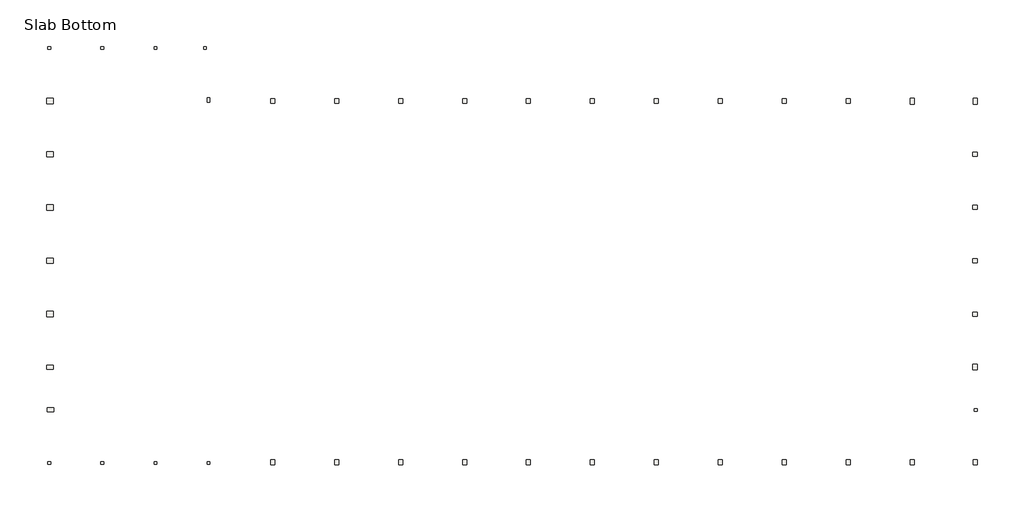
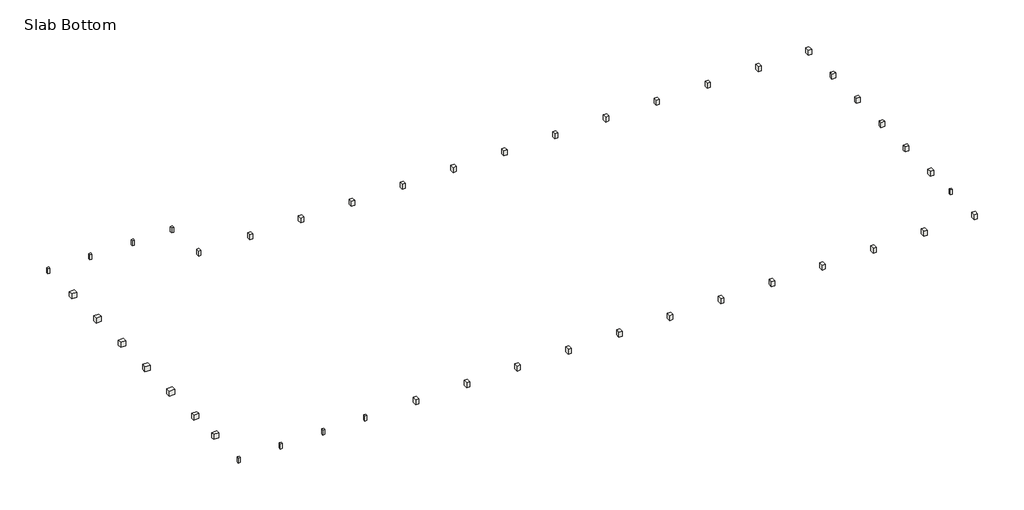
# One storey: 46 slabs.
"""IFC4 building model written with IfcOpenShell, lengths in millimetres."""

from ifc_helpers import new_model, si_unit, frame, origin, place, context, project, spatial, polyline, outline, extrude, element, save

model = new_model("IFC4")

# Units and contexts
model_context = context("Model", 3, world=origin())
ifc_project = project(units=[si_unit("LENGTHUNIT", "METRE", prefix="MILLI")], contexts=[model_context])

# Site, building, storey
site = spatial("IfcSite", under=ifc_project)
building = spatial("IfcBuilding", under=site)
storey = spatial("IfcBuildingStorey", under=building, Name="Slab Bottom", Elevation=-152.4)

# Slabs
placement = place(None, origin())
element("IfcSlab", 1, ObjectType="Footing-Rectangular : P1", at=placement, inside=storey, context=model_context, shape_type="SweptSolid", body=[
    extrude(outline(polyline([(304747.7148264, -530797.8413841), (305052.5148264, -530797.8413841), (305052.5148264, -531102.6413841), (304747.7148264, -531102.6413841), (304747.7148264, -530797.8413841)])), frame((0.0, 0.0, -1066.8), z_axis=(0.0, 0.0, 1.0), x_axis=(1.0, 0.0, 0.0)), (0.0, 0.0, 1.0), 762.0),
])
element("IfcSlab", 2, ObjectType="Footing-Rectangular : P1", at=placement, inside=storey, context=model_context, shape_type="SweptSolid", body=[
    extrude(outline(polyline([(310840.5398264, -530801.0163841), (311145.3398264, -530801.0163841), (311145.3398264, -531105.8163841), (310840.5398264, -531105.8163841), (310840.5398264, -530801.0163841)])), frame((0.0, 0.0, -1066.8), z_axis=(0.0, 0.0, 1.0), x_axis=(1.0, 0.0, 0.0)), (0.0, 0.0, 1.0), 762.0),
])
element("IfcSlab", 3, ObjectType="Footing-Rectangular : P1", at=placement, inside=storey, context=model_context, shape_type="SweptSolid", body=[
    extrude(outline(polyline([(316968.2898264, -530801.0163841), (317273.0898264, -530801.0163841), (317273.0898264, -531105.8163841), (316968.2898264, -531105.8163841), (316968.2898264, -530801.0163841)])), frame((0.0, 0.0, -1066.8), z_axis=(0.0, 0.0, 1.0), x_axis=(1.0, 0.0, 0.0)), (0.0, 0.0, 1.0), 762.0),
])
element("IfcSlab", 4, ObjectType="Footing-Rectangular : P1", at=placement, inside=storey, context=model_context, shape_type="SweptSolid", body=[
    extrude(outline(polyline([(322661.0648264, -531102.6413841), (322661.0648264, -530797.8413841), (322965.8648264, -530797.8413841), (322965.8648264, -531102.6413841), (322661.0648264, -531102.6413841)])), frame((0.0, 0.0, -1066.8), z_axis=(0.0, 0.0, 1.0), x_axis=(1.0, 0.0, 0.0)), (0.0, 0.0, 1.0), 762.0),
])
element("IfcSlab", 5, ObjectType="Footing-Rectangular : P1", at=placement, inside=storey, context=model_context, shape_type="SweptSolid", body=[
    extrude(outline(polyline([(304741.3648264, -578543.4913841), (305046.1648264, -578543.4913841), (305046.1648264, -578848.2913841), (304741.3648264, -578848.2913841), (304741.3648264, -578543.4913841)])), frame((0.0, 0.0, -1066.8), z_axis=(0.0, 0.0, 1.0), x_axis=(1.0, 0.0, 0.0)), (0.0, 0.0, 1.0), 762.0),
])
element("IfcSlab", 6, ObjectType="Footing-Rectangular : P1", at=placement, inside=storey, context=model_context, shape_type="SweptSolid", body=[
    extrude(outline(polyline([(310840.5398264, -578845.1163841), (310840.5398264, -578540.3163841), (311145.3398264, -578540.3163841), (311145.3398264, -578845.1163841), (310840.5398264, -578845.1163841)])), frame((0.0, 0.0, -1066.8), z_axis=(0.0, 0.0, 1.0), x_axis=(1.0, 0.0, 0.0)), (0.0, 0.0, 1.0), 762.0),
])
element("IfcSlab", 7, ObjectType="Footing-Rectangular : P1", at=placement, inside=storey, context=model_context, shape_type="SweptSolid", body=[
    extrude(outline(polyline([(316971.4648264, -578845.1163841), (316971.4648264, -578540.3163841), (317276.2648264, -578540.3163841), (317276.2648264, -578845.1163841), (316971.4648264, -578845.1163841)])), frame((0.0, 0.0, -1066.8), z_axis=(0.0, 0.0, 1.0), x_axis=(1.0, 0.0, 0.0)), (0.0, 0.0, 1.0), 762.0),
])
element("IfcSlab", 8, ObjectType="Footing-Rectangular : P1", at=placement, inside=storey, context=model_context, shape_type="SweptSolid", body=[
    extrude(outline(polyline([(323067.4648264, -578543.4913841), (323372.2648264, -578543.4913841), (323372.2648264, -578848.2913841), (323067.4648264, -578848.2913841), (323067.4648264, -578543.4913841)])), frame((0.0, 0.0, -1066.8), z_axis=(0.0, 0.0, 1.0), x_axis=(1.0, 0.0, 0.0)), (0.0, 0.0, 1.0), 762.0),
])
element("IfcSlab", 9, ObjectType="Footing-Rectangular : P1", at=placement, inside=storey, context=model_context, shape_type="SweptSolid", body=[
    extrude(outline(polyline([(411307.0648264, -572441.1413841), (411611.8648264, -572441.1413841), (411611.8648264, -572745.9413841), (411307.0648264, -572745.9413841), (411307.0648264, -572441.1413841)])), frame((0.0, 0.0, -1066.8), z_axis=(0.0, 0.0, 1.0), x_axis=(1.0, 0.0, 0.0)), (0.0, 0.0, 1.0), 762.0),
])
element("IfcSlab", 10, ObjectType="Footing-Rectangular : P2", at=placement, inside=storey, context=model_context, shape_type="SweptSolid", body=[
    extrude(outline(polyline([(323375.4398264, -536716.0413841), (323375.4398264, -537224.0413841), (323070.6398264, -537224.0413841), (323070.6398264, -536716.0413841), (323375.4398264, -536716.0413841)])), frame((0.0, 0.0, -1066.8), z_axis=(0.0, 0.0, 1.0), x_axis=(1.0, 0.0, 0.0)), (0.0, 0.0, 1.0), 762.0),
])
element("IfcSlab", 11, ObjectType="Footing-Rectangular : P3", at=placement, inside=storey, context=model_context, shape_type="SweptSolid", body=[
    extrude(outline(polyline([(411110.2148264, -561334.9913841), (411643.6148264, -561334.9913841), (411643.6148264, -561792.1913841), (411110.2148264, -561792.1913841), (411110.2148264, -561334.9913841)])), frame((0.0, 0.0, -1066.8), z_axis=(0.0, 0.0, 1.0), x_axis=(1.0, 0.0, 0.0)), (0.0, 0.0, 1.0), 762.0),
])
element("IfcSlab", 12, ObjectType="Footing-Rectangular : P3", at=placement, inside=storey, context=model_context, shape_type="SweptSolid", body=[
    extrude(outline(polyline([(411110.2148264, -555207.2413841), (411643.6148264, -555207.2413841), (411643.6148264, -555664.4413841), (411110.2148264, -555664.4413841), (411110.2148264, -555207.2413841)])), frame((0.0, 0.0, -1066.8), z_axis=(0.0, 0.0, 1.0), x_axis=(1.0, 0.0, 0.0)), (0.0, 0.0, 1.0), 762.0),
])
element("IfcSlab", 13, ObjectType="Footing-Rectangular : P3", at=placement, inside=storey, context=model_context, shape_type="SweptSolid", body=[
    extrude(outline(polyline([(411110.2148264, -549079.4913841), (411643.6148264, -549079.4913841), (411643.6148264, -549536.6913841), (411110.2148264, -549536.6913841), (411110.2148264, -549079.4913841)])), frame((0.0, 0.0, -1066.8), z_axis=(0.0, 0.0, 1.0), x_axis=(1.0, 0.0, 0.0)), (0.0, 0.0, 1.0), 762.0),
])
element("IfcSlab", 14, ObjectType="Footing-Rectangular : P3", at=placement, inside=storey, context=model_context, shape_type="SweptSolid", body=[
    extrude(outline(polyline([(411110.2148264, -542951.7413841), (411643.6148264, -542951.7413841), (411643.6148264, -543408.9413841), (411110.2148264, -543408.9413841), (411110.2148264, -542951.7413841)])), frame((0.0, 0.0, -1066.8), z_axis=(0.0, 0.0, 1.0), x_axis=(1.0, 0.0, 0.0)), (0.0, 0.0, 1.0), 762.0),
])
element("IfcSlab", 15, ObjectType="Footing-Rectangular : P3A", at=placement, inside=storey, context=model_context, shape_type="SweptSolid", body=[
    extrude(outline(polyline([(397010.0398264, -536811.2913841), (397010.0398264, -537344.6913841), (396552.8398264, -537344.6913841), (396552.8398264, -536811.2913841), (397010.0398264, -536811.2913841)])), frame((0.0, 0.0, -1066.8), z_axis=(0.0, 0.0, 1.0), x_axis=(1.0, 0.0, 0.0)), (0.0, 0.0, 1.0), 762.0),
])
element("IfcSlab", 16, ObjectType="Footing-Rectangular : P3A", at=placement, inside=storey, context=model_context, shape_type="SweptSolid", body=[
    extrude(outline(polyline([(389656.7398264, -536811.2913841), (389656.7398264, -537344.6913841), (389199.5398264, -537344.6913841), (389199.5398264, -536811.2913841), (389656.7398264, -536811.2913841)])), frame((0.0, 0.0, -1066.8), z_axis=(0.0, 0.0, 1.0), x_axis=(1.0, 0.0, 0.0)), (0.0, 0.0, 1.0), 762.0),
])
element("IfcSlab", 17, ObjectType="Footing-Rectangular : P3A", at=placement, inside=storey, context=model_context, shape_type="SweptSolid", body=[
    extrude(outline(polyline([(382303.4398264, -536811.2913841), (382303.4398264, -537344.6913841), (381846.2398264, -537344.6913841), (381846.2398264, -536811.2913841), (382303.4398264, -536811.2913841)])), frame((0.0, 0.0, -1066.8), z_axis=(0.0, 0.0, 1.0), x_axis=(1.0, 0.0, 0.0)), (0.0, 0.0, 1.0), 762.0),
])
element("IfcSlab", 18, ObjectType="Footing-Rectangular : P3A", at=placement, inside=storey, context=model_context, shape_type="SweptSolid", body=[
    extrude(outline(polyline([(374950.1398264, -536811.2913841), (374950.1398264, -537344.6913841), (374492.9398264, -537344.6913841), (374492.9398264, -536811.2913841), (374950.1398264, -536811.2913841)])), frame((0.0, 0.0, -1066.8), z_axis=(0.0, 0.0, 1.0), x_axis=(1.0, 0.0, 0.0)), (0.0, 0.0, 1.0), 762.0),
])
element("IfcSlab", 19, ObjectType="Footing-Rectangular : P3A", at=placement, inside=storey, context=model_context, shape_type="SweptSolid", body=[
    extrude(outline(polyline([(367596.8398264, -536811.2913841), (367596.8398264, -537344.6913841), (367139.6398264, -537344.6913841), (367139.6398264, -536811.2913841), (367596.8398264, -536811.2913841)])), frame((0.0, 0.0, -1066.8), z_axis=(0.0, 0.0, 1.0), x_axis=(1.0, 0.0, 0.0)), (0.0, 0.0, 1.0), 762.0),
])
element("IfcSlab", 20, ObjectType="Footing-Rectangular : P3A", at=placement, inside=storey, context=model_context, shape_type="SweptSolid", body=[
    extrude(outline(polyline([(360243.5398264, -536811.2913841), (360243.5398264, -537344.6913841), (359786.3398264, -537344.6913841), (359786.3398264, -536811.2913841), (360243.5398264, -536811.2913841)])), frame((0.0, 0.0, -1066.8), z_axis=(0.0, 0.0, 1.0), x_axis=(1.0, 0.0, 0.0)), (0.0, 0.0, 1.0), 762.0),
])
element("IfcSlab", 21, ObjectType="Footing-Rectangular : P3A", at=placement, inside=storey, context=model_context, shape_type="SweptSolid", body=[
    extrude(outline(polyline([(352890.2398264, -536811.2913841), (352890.2398264, -537344.6913841), (352433.0398264, -537344.6913841), (352433.0398264, -536811.2913841), (352890.2398264, -536811.2913841)])), frame((0.0, 0.0, -1066.8), z_axis=(0.0, 0.0, 1.0), x_axis=(1.0, 0.0, 0.0)), (0.0, 0.0, 1.0), 762.0),
])
element("IfcSlab", 22, ObjectType="Footing-Rectangular : P3A", at=placement, inside=storey, context=model_context, shape_type="SweptSolid", body=[
    extrude(outline(polyline([(345536.9398264, -536811.2913841), (345536.9398264, -537344.6913841), (345079.7398264, -537344.6913841), (345079.7398264, -536811.2913841), (345536.9398264, -536811.2913841)])), frame((0.0, 0.0, -1066.8), z_axis=(0.0, 0.0, 1.0), x_axis=(1.0, 0.0, 0.0)), (0.0, 0.0, 1.0), 762.0),
])
element("IfcSlab", 23, ObjectType="Footing-Rectangular : P3A", at=placement, inside=storey, context=model_context, shape_type="SweptSolid", body=[
    extrude(outline(polyline([(338183.6398264, -536811.2913841), (338183.6398264, -537344.6913841), (337726.4398264, -537344.6913841), (337726.4398264, -536811.2913841), (338183.6398264, -536811.2913841)])), frame((0.0, 0.0, -1066.8), z_axis=(0.0, 0.0, 1.0), x_axis=(1.0, 0.0, 0.0)), (0.0, 0.0, 1.0), 762.0),
])
element("IfcSlab", 24, ObjectType="Footing-Rectangular : P3A", at=placement, inside=storey, context=model_context, shape_type="SweptSolid", body=[
    extrude(outline(polyline([(330830.3398264, -536811.2913841), (330830.3398264, -537344.6913841), (330373.1398264, -537344.6913841), (330373.1398264, -536811.2913841), (330830.3398264, -536811.2913841)])), frame((0.0, 0.0, -1066.8), z_axis=(0.0, 0.0, 1.0), x_axis=(1.0, 0.0, 0.0)), (0.0, 0.0, 1.0), 762.0),
])
element("IfcSlab", 25, ObjectType="Footing-Rectangular : P4", at=placement, inside=storey, context=model_context, shape_type="SweptSolid", body=[
    extrude(outline(polyline([(330830.3398264, -578318.0663841), (330830.3398264, -578927.6663841), (330373.1398264, -578927.6663841), (330373.1398264, -578318.0663841), (330830.3398264, -578318.0663841)])), frame((0.0, 0.0, -1066.8), z_axis=(0.0, 0.0, 1.0), x_axis=(1.0, 0.0, 0.0)), (0.0, 0.0, 1.0), 762.0),
])
element("IfcSlab", 26, ObjectType="Footing-Rectangular : P4", at=placement, inside=storey, context=model_context, shape_type="SweptSolid", body=[
    extrude(outline(polyline([(338183.6398264, -578318.0663841), (338183.6398264, -578927.6663841), (337726.4398264, -578927.6663841), (337726.4398264, -578318.0663841), (338183.6398264, -578318.0663841)])), frame((0.0, 0.0, -1066.8), z_axis=(0.0, 0.0, 1.0), x_axis=(1.0, 0.0, 0.0)), (0.0, 0.0, 1.0), 762.0),
])
element("IfcSlab", 27, ObjectType="Footing-Rectangular : P4", at=placement, inside=storey, context=model_context, shape_type="SweptSolid", body=[
    extrude(outline(polyline([(345536.9398264, -578318.0663841), (345536.9398264, -578927.6663841), (345079.7398264, -578927.6663841), (345079.7398264, -578318.0663841), (345536.9398264, -578318.0663841)])), frame((0.0, 0.0, -1066.8), z_axis=(0.0, 0.0, 1.0), x_axis=(1.0, 0.0, 0.0)), (0.0, 0.0, 1.0), 762.0),
])
element("IfcSlab", 28, ObjectType="Footing-Rectangular : P4", at=placement, inside=storey, context=model_context, shape_type="SweptSolid", body=[
    extrude(outline(polyline([(352890.2398264, -578318.0663841), (352890.2398264, -578927.6663841), (352433.0398264, -578927.6663841), (352433.0398264, -578318.0663841), (352890.2398264, -578318.0663841)])), frame((0.0, 0.0, -1066.8), z_axis=(0.0, 0.0, 1.0), x_axis=(1.0, 0.0, 0.0)), (0.0, 0.0, 1.0), 762.0),
])
element("IfcSlab", 29, ObjectType="Footing-Rectangular : P4", at=placement, inside=storey, context=model_context, shape_type="SweptSolid", body=[
    extrude(outline(polyline([(360243.5398264, -578318.0663841), (360243.5398264, -578927.6663841), (359786.3398264, -578927.6663841), (359786.3398264, -578318.0663841), (360243.5398264, -578318.0663841)])), frame((0.0, 0.0, -1066.8), z_axis=(0.0, 0.0, 1.0), x_axis=(1.0, 0.0, 0.0)), (0.0, 0.0, 1.0), 762.0),
])
element("IfcSlab", 30, ObjectType="Footing-Rectangular : P4", at=placement, inside=storey, context=model_context, shape_type="SweptSolid", body=[
    extrude(outline(polyline([(367596.8398264, -578318.0663841), (367596.8398264, -578927.6663841), (367139.6398264, -578927.6663841), (367139.6398264, -578318.0663841), (367596.8398264, -578318.0663841)])), frame((0.0, 0.0, -1066.8), z_axis=(0.0, 0.0, 1.0), x_axis=(1.0, 0.0, 0.0)), (0.0, 0.0, 1.0), 762.0),
])
element("IfcSlab", 31, ObjectType="Footing-Rectangular : P4", at=placement, inside=storey, context=model_context, shape_type="SweptSolid", body=[
    extrude(outline(polyline([(374950.1398264, -578318.0663841), (374950.1398264, -578927.6663841), (374492.9398264, -578927.6663841), (374492.9398264, -578318.0663841), (374950.1398264, -578318.0663841)])), frame((0.0, 0.0, -1066.8), z_axis=(0.0, 0.0, 1.0), x_axis=(1.0, 0.0, 0.0)), (0.0, 0.0, 1.0), 762.0),
])
element("IfcSlab", 32, ObjectType="Footing-Rectangular : P4", at=placement, inside=storey, context=model_context, shape_type="SweptSolid", body=[
    extrude(outline(polyline([(382303.4398264, -578318.0663841), (382303.4398264, -578927.6663841), (381846.2398264, -578927.6663841), (381846.2398264, -578318.0663841), (382303.4398264, -578318.0663841)])), frame((0.0, 0.0, -1066.8), z_axis=(0.0, 0.0, 1.0), x_axis=(1.0, 0.0, 0.0)), (0.0, 0.0, 1.0), 762.0),
])
element("IfcSlab", 33, ObjectType="Footing-Rectangular : P4", at=placement, inside=storey, context=model_context, shape_type="SweptSolid", body=[
    extrude(outline(polyline([(389656.7398264, -578318.0663841), (389656.7398264, -578927.6663841), (389199.5398264, -578927.6663841), (389199.5398264, -578318.0663841), (389656.7398264, -578318.0663841)])), frame((0.0, 0.0, -1066.8), z_axis=(0.0, 0.0, 1.0), x_axis=(1.0, 0.0, 0.0)), (0.0, 0.0, 1.0), 762.0),
])
element("IfcSlab", 34, ObjectType="Footing-Rectangular : P4", at=placement, inside=storey, context=model_context, shape_type="SweptSolid", body=[
    extrude(outline(polyline([(397010.0398264, -578311.7163841), (397010.0398264, -578921.3163841), (396552.8398264, -578921.3163841), (396552.8398264, -578311.7163841), (397010.0398264, -578311.7163841)])), frame((0.0, 0.0, -1066.8), z_axis=(0.0, 0.0, 1.0), x_axis=(1.0, 0.0, 0.0)), (0.0, 0.0, 1.0), 762.0),
])
element("IfcSlab", 35, ObjectType="Footing-Rectangular : P4A", at=placement, inside=storey, context=model_context, shape_type="SweptSolid", body=[
    extrude(outline(polyline([(404363.3398264, -578311.7163841), (404363.3398264, -578921.3163841), (403906.1398264, -578921.3163841), (403906.1398264, -578311.7163841), (404363.3398264, -578311.7163841)])), frame((0.0, 0.0, -1066.8), z_axis=(0.0, 0.0, 1.0), x_axis=(1.0, 0.0, 0.0)), (0.0, 0.0, 1.0), 762.0),
])
element("IfcSlab", 36, ObjectType="Footing-Rectangular : P4A", at=placement, inside=storey, context=model_context, shape_type="SweptSolid", body=[
    extrude(outline(polyline([(411659.4898264, -578311.7163841), (411659.4898264, -578921.3163841), (411202.2898264, -578921.3163841), (411202.2898264, -578311.7163841), (411659.4898264, -578311.7163841)])), frame((0.0, 0.0, -1066.8), z_axis=(0.0, 0.0, 1.0), x_axis=(1.0, 0.0, 0.0)), (0.0, 0.0, 1.0), 762.0),
])
element("IfcSlab", 37, ObjectType="Footing-Rectangular : P5", at=placement, inside=storey, context=model_context, shape_type="SweptSolid", body=[
    extrude(outline(polyline([(411615.0397781, -536747.7913841), (411615.0397781, -537408.1913841), (411157.8397781, -537408.1913841), (411157.8397781, -536747.7913841), (411615.0397781, -536747.7913841)])), frame((0.0, 0.0, -1066.8), z_axis=(0.0, 0.0, 1.0), x_axis=(1.0, 0.0, 0.0)), (0.0, 0.0, 1.0), 762.0),
])
element("IfcSlab", 38, ObjectType="Footing-Rectangular : P5", at=placement, inside=storey, context=model_context, shape_type="SweptSolid", body=[
    extrude(outline(polyline([(404363.3398264, -536747.7913841), (404363.3398264, -537408.1913841), (403906.1398264, -537408.1913841), (403906.1398264, -536747.7913841), (404363.3398264, -536747.7913841)])), frame((0.0, 0.0, -1066.8), z_axis=(0.0, 0.0, 1.0), x_axis=(1.0, 0.0, 0.0)), (0.0, 0.0, 1.0), 762.0),
])
element("IfcSlab", 39, ObjectType="Footing-Rectangular : P6", at=placement, inside=storey, context=model_context, shape_type="SweptSolid", body=[
    extrude(outline(polyline([(304642.9398264, -572364.9413841), (305404.9398264, -572364.9413841), (305404.9398264, -572822.1413841), (304642.9398264, -572822.1413841), (304642.9398264, -572364.9413841)])), frame((0.0, 0.0, -1066.8), z_axis=(0.0, 0.0, 1.0), x_axis=(1.0, 0.0, 0.0)), (0.0, 0.0, 1.0), 762.0),
])
element("IfcSlab", 40, ObjectType="Footing-Rectangular : P6A", at=placement, inside=storey, context=model_context, shape_type="SweptSolid", body=[
    extrude(outline(polyline([(304585.7898264, -567462.7413841), (305347.7898264, -567462.7413841), (305347.7898264, -567919.9413841), (304585.7898264, -567919.9413841), (304585.7898264, -567462.7413841)])), frame((0.0, 0.0, -1066.8), z_axis=(0.0, 0.0, 1.0), x_axis=(1.0, 0.0, 0.0)), (0.0, 0.0, 1.0), 762.0),
])
element("IfcSlab", 41, ObjectType="Footing-Rectangular : P7", at=placement, inside=storey, context=model_context, shape_type="SweptSolid", body=[
    extrude(outline(polyline([(411640.4398264, -567361.1414082), (411640.4398264, -567970.7414082), (411132.4398264, -567970.7414082), (411132.4398264, -567361.1414082), (411640.4398264, -567361.1414082)])), frame((0.0, 0.0, -1066.8), z_axis=(0.0, 0.0, 1.0), x_axis=(1.0, 0.0, 0.0)), (0.0, 0.0, 1.0), 762.0),
])
element("IfcSlab", 42, ObjectType="Footing-Rectangular : P8", at=placement, inside=storey, context=model_context, shape_type="SweptSolid", body=[
    extrude(outline(polyline([(304585.7898264, -536747.7913841), (305347.7898264, -536747.7913841), (305347.7898264, -537357.3913841), (304585.7898264, -537357.3913841), (304585.7898264, -536747.7913841)])), frame((0.0, 0.0, -1066.8), z_axis=(0.0, 0.0, 1.0), x_axis=(1.0, 0.0, 0.0)), (0.0, 0.0, 1.0), 762.0),
])
element("IfcSlab", 43, ObjectType="Footing-Rectangular : P8", at=placement, inside=storey, context=model_context, shape_type="SweptSolid", body=[
    extrude(outline(polyline([(304585.7898264, -542875.5413841), (305347.7898264, -542875.5413841), (305347.7898264, -543485.1413841), (304585.7898264, -543485.1413841), (304585.7898264, -542875.5413841)])), frame((0.0, 0.0, -1066.8), z_axis=(0.0, 0.0, 1.0), x_axis=(1.0, 0.0, 0.0)), (0.0, 0.0, 1.0), 762.0),
])
element("IfcSlab", 44, ObjectType="Footing-Rectangular : P8", at=placement, inside=storey, context=model_context, shape_type="SweptSolid", body=[
    extrude(outline(polyline([(304585.7898264, -549003.2913841), (305347.7898264, -549003.2913841), (305347.7898264, -549612.8913841), (304585.7898264, -549612.8913841), (304585.7898264, -549003.2913841)])), frame((0.0, 0.0, -1066.8), z_axis=(0.0, 0.0, 1.0), x_axis=(1.0, 0.0, 0.0)), (0.0, 0.0, 1.0), 762.0),
])
element("IfcSlab", 45, ObjectType="Footing-Rectangular : P8", at=placement, inside=storey, context=model_context, shape_type="SweptSolid", body=[
    extrude(outline(polyline([(304585.7898264, -555131.0413841), (305347.7898264, -555131.0413841), (305347.7898264, -555740.6413841), (304585.7898264, -555740.6413841), (304585.7898264, -555131.0413841)])), frame((0.0, 0.0, -1066.8), z_axis=(0.0, 0.0, 1.0), x_axis=(1.0, 0.0, 0.0)), (0.0, 0.0, 1.0), 762.0),
])
element("IfcSlab", 46, ObjectType="Footing-Rectangular : P8", at=placement, inside=storey, context=model_context, shape_type="SweptSolid", body=[
    extrude(outline(polyline([(304585.7898264, -561258.7913841), (305347.7898264, -561258.7913841), (305347.7898264, -561868.3913841), (304585.7898264, -561868.3913841), (304585.7898264, -561258.7913841)])), frame((0.0, 0.0, -1066.8), z_axis=(0.0, 0.0, 1.0), x_axis=(1.0, 0.0, 0.0)), (0.0, 0.0, 1.0), 762.0),
])

save(model, "model.ifc")

# Revit data of these elements
# Type "Footing-Rectangular : P1"
#   Type Mark = ""
#   Assembly Code = "A1010100"
#   Width = 1' - 0"
#   Length = 1' - 0"
#   Thickness = 2' - 6"
#   Structural Material [instance default] = Concrete, Cast-in-Place gray
# Type "Footing-Rectangular : P2"
#   Assembly Code = "A1010100"
#   Width = 1' - 0"
#   Length = 1' - 8"
#   Thickness = 2' - 6"
#   Structural Material [instance default] = Concrete, Cast-in-Place gray
# Type "Footing-Rectangular : P3"
#   Assembly Code = "A1010100"
#   Width = 1' - 6"
#   Length = 1' - 9"
#   Thickness = 2' - 6"
#   Structural Material [instance default] = Concrete, Cast-in-Place gray
# Type "Footing-Rectangular : P3A"
#   Assembly Code = "A1010100"
#   Width = 1' - 6"
#   Length = 1' - 9"
#   Thickness = 2' - 6"
#   Structural Material [instance default] = Concrete, Cast-in-Place gray
# Type "Footing-Rectangular : P4"
#   Assembly Code = "A1010100"
#   Width = 1' - 6"
#   Length = 2' - 0"
#   Thickness = 2' - 6"
#   Structural Material [instance default] = Concrete, Cast-in-Place gray
# Type "Footing-Rectangular : P4A"
#   Assembly Code = "A1010100"
#   Width = 1' - 6"
#   Length = 2' - 0"
#   Thickness = 2' - 6"
#   Structural Material [instance default] = Concrete, Cast-in-Place gray
# Type "Footing-Rectangular : P5"
#   Assembly Code = "A1010100"
#   Width = 1' - 6"
#   Length = 2' - 2"
#   Thickness = 2' - 6"
#   Structural Material [instance default] = Concrete, Cast-in-Place gray
# Type "Footing-Rectangular : P6"
#   Assembly Code = "A1010100"
#   Width = 1' - 6"
#   Length = 2' - 6"
#   Thickness = 2' - 6"
#   Structural Material [instance default] = Concrete, Cast-in-Place gray
# Type "Footing-Rectangular : P6A"
#   Assembly Code = "A1010100"
#   Width = 1' - 6"
#   Length = 2' - 6"
#   Thickness = 2' - 6"
#   Structural Material [instance default] = Concrete, Cast-in-Place gray
# Type "Footing-Rectangular : P7"
#   Assembly Code = "A1010100"
#   Width = 1' - 8"
#   Length = 2' - 0"
#   Thickness = 2' - 6"
#   Structural Material [instance default] = Concrete, Cast-in-Place gray
# Type "Footing-Rectangular : P8"
#   Assembly Code = "A1010100"
#   Width = 2' - 0"
#   Length = 2' - 6"
#   Thickness = 2' - 6"
#   Structural Material [instance default] = Concrete, Cast-in-Place gray
# Elements 1, 2, 3, 4, 5, 6, 7, 8, 9 (IfcSlab, "Footing-Rectangular : P1")
#   Comments = ""
#   Structural Material = Concrete, Cast-in-Place gray
#   Phase Created = New Construction
#   Materials on its faces: "Concrete, Cast-in-Place gray"
# Element 10 (IfcSlab, "Footing-Rectangular : P2")
#   Comments = ""
#   Structural Material = Concrete, Cast-in-Place gray
#   Phase Created = New Construction
#   Materials on its faces: "Concrete, Cast-in-Place gray"
# Elements 11, 12, 13, 14 (IfcSlab, "Footing-Rectangular : P3")
#   Comments = ""
#   Structural Material = Concrete, Cast-in-Place gray
#   Phase Created = New Construction
#   Materials on its faces: "Concrete, Cast-in-Place gray"
# Elements 15, 16, 17, 18, 19, 20, 21, 22, 23, 24 (IfcSlab, "Footing-Rectangular : P3A")
#   Comments = ""
#   Structural Material = Concrete, Cast-in-Place gray
#   Phase Created = New Construction
#   Materials on its faces: "Concrete, Cast-in-Place gray"
# Elements 25, 26, 27, 28, 29, 30, 31, 32, 33, 34 (IfcSlab, "Footing-Rectangular : P4")
#   Comments = ""
#   Structural Material = Concrete, Cast-in-Place gray
#   Phase Created = New Construction
#   Materials on its faces: "Concrete, Cast-in-Place gray"
# Elements 35, 36 (IfcSlab, "Footing-Rectangular : P4A")
#   Comments = ""
#   Structural Material = Concrete, Cast-in-Place gray
#   Phase Created = New Construction
#   Materials on its faces: "Concrete, Cast-in-Place gray"
# Elements 37, 38 (IfcSlab, "Footing-Rectangular : P5")
#   Comments = ""
#   Structural Material = Concrete, Cast-in-Place gray
#   Phase Created = New Construction
#   Materials on its faces: "Concrete, Cast-in-Place gray"
# Element 39 (IfcSlab, "Footing-Rectangular : P6")
#   Comments = ""
#   Structural Material = Concrete, Cast-in-Place gray
#   Phase Created = New Construction
#   Materials on its faces: "Concrete, Cast-in-Place gray"
# Element 40 (IfcSlab, "Footing-Rectangular : P6A")
#   Comments = ""
#   Structural Material = Concrete, Cast-in-Place gray
#   Phase Created = New Construction
#   Materials on its faces: "Concrete, Cast-in-Place gray"
# Element 41 (IfcSlab, "Footing-Rectangular : P7")
#   Comments = ""
#   Structural Material = Concrete, Cast-in-Place gray
#   Phase Created = New Construction
#   Materials on its faces: "Concrete, Cast-in-Place gray"
# Elements 42, 43, 44, 45, 46 (IfcSlab, "Footing-Rectangular : P8")
#   Comments = ""
#   Structural Material = Concrete, Cast-in-Place gray
#   Phase Created = New Construction
#   Materials on its faces: "Concrete, Cast-in-Place gray"
# Materials
#   "Concrete, Cast-in-Place gray": class "Concrete", colour RGB 192 192 192, transparency 0, Description = "Cast-in-place concrete", Cost = 0
